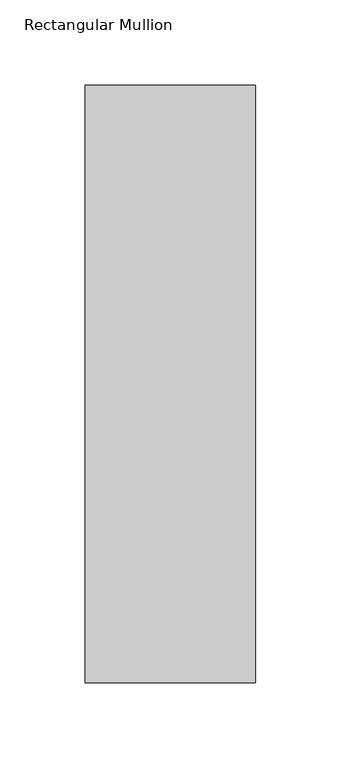
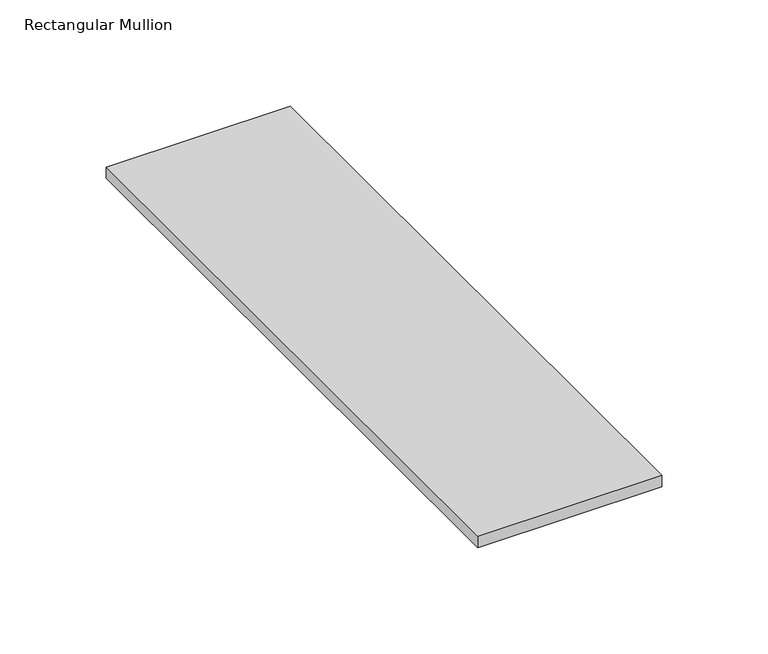
"""IFC4 building model written with IfcOpenShell, lengths in millimetres: member geometry, Rectangular Mullion : WWm-100x350-100mmOffset."""

from ifc_helpers import new_model, si_unit, frame, origin, place, context, project, spatial, polyline, outline, extrude, source, transform, mapped, element, save


def rectangular_mullion_85b2d351(model_context):
    return source(origin(), model_context, "Body", "SweptSolid", [
        extrude(outline(polyline([(0.0, 175.0), (0.0, -175.0), (-100.0, -175.0), (-100.0, 175.0), (0.0, 175.0)])), frame((0.0, 0.0, -6.4680799), z_axis=(0.0, 0.0, 1.0), x_axis=(1.0, 0.0, 0.0)), (0.0, 0.0, 1.0), 6.4680799),
    ])


if __name__ == "__main__":
    model = new_model("IFC4")
    model_context = context("Model", 3, world=origin())
    ifc_project = project(units=[si_unit("LENGTHUNIT", "METRE", prefix="MILLI")], contexts=[model_context])
    site = spatial("IfcSite", under=ifc_project)
    building = spatial("IfcBuilding", under=site)
    placement = place(None, origin())
    rectangular_mullion_shape = rectangular_mullion_85b2d351(model_context)
    element("IfcMember", 1, ObjectType="Rectangular Mullion : WWm-100x350-100mmOffset", at=placement, inside=building, context=model_context, shape_type="MappedRepresentation", body=[
        mapped(rectangular_mullion_shape, transform((0.0, 0.0, 0.0), x_axis=(1.0, 0.0, 0.0), y_axis=(0.0, 1.0, 0.0), z_axis=(0.0, 0.0, 1.0))),
    ])
    save(model, "model.ifc")

# Revit data of these elements
# Type "Rectangular Mullion : WWm-100x350-100mmOffset"
#   built-in parameter 1007304 = 1.14829 (stored number, unit not read)
#   built-in parameter 1007301 = 0.164042 (stored number, unit not read)
#   built-in parameter 1007300 = 0.164042 (stored number, unit not read)
# Element 1 (IfcMember, "Rectangular Mullion : WWm-100x350-100mmOffset")
#   Materials on its faces: "WW-EC-RGB-Mullion"
# Materials
#   "WW-EC-RGB-Mullion": class "Generic", colour RGB 255 255 255, transparency 0, Comments = "If region requests black mullions, switch asset color to RGB 25-25-25", Description = "Generic Color", Cost = 0
